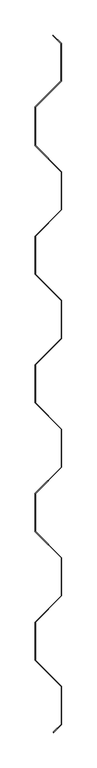
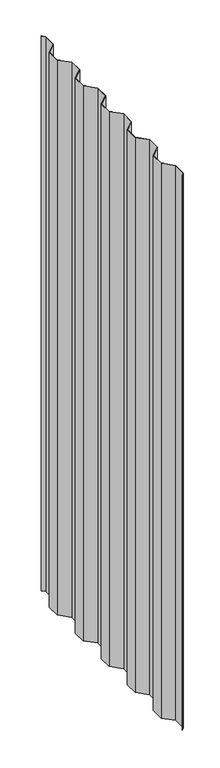
"""IFC4 building model written with IfcOpenShell, lengths in millimetres: proxy geometry, MBCI 7.2-V Panel7 : MBCI 7.2-V Panel-1."""

from ifc_helpers import new_model, si_unit, frame, origin, place, context, project, spatial, polyline, outline, extrude, source, transform, mapped, element, save


def generic_models_abe479ed(model_context):
    return source(origin(), model_context, "Body", "SweptSolid", [
        extrude(outline(polyline([(587365.8648989, -532709.4731976), (587365.8648989, -532763.5849068), (587354.4642648, -532774.9855409), (587354.4223399, -532774.1855668), (587365.2695864, -532763.3383203), (587365.2695864, -532709.7197841), (587327.7791864, -532672.2293841), (587327.7791864, -532617.9487203), (587365.2695864, -532580.4583203), (587365.2695864, -532526.8397841), (587327.7791864, -532489.3493841), (587327.7791864, -532435.0687203), (587365.2695864, -532397.5783203), (587365.2695864, -532343.9597841), (587327.7791864, -532306.4693841), (587327.7791864, -532252.1887203), (587365.2695864, -532214.6983203), (587365.2695864, -532161.0797841), (587327.7791864, -532123.5893841), (587327.7791864, -532069.3087203), (587365.2695864, -532031.8183203), (587365.2695864, -531978.1997841), (587327.7791864, -531940.7093841), (587327.7791864, -531885.5651203), (587364.6599864, -531848.6843203), (587364.6599864, -531795.5961933), (587353.5295525, -531784.4657594), (587353.5845762, -531783.6788841), (587365.2552989, -531795.3496068), (587365.2552989, -531848.9309068), (587328.3744989, -531885.8117068), (587328.3744989, -531940.4627976), (587365.8648989, -531977.9531976), (587365.8648989, -532032.0649068), (587328.3744989, -532069.5553068), (587328.3744989, -532123.3427976), (587365.8648989, -532160.8331976), (587365.8648989, -532214.9449068), (587328.3744989, -532252.4353068), (587328.3744989, -532306.2227976), (587365.8648989, -532343.7131976), (587365.8648989, -532397.8249068), (587328.3744989, -532435.3153068), (587328.3744989, -532489.1027976), (587365.8648989, -532526.5931976), (587365.8648989, -532580.7049068), (587328.3744989, -532618.1953068), (587328.3744989, -532671.9827976), (587365.8648989, -532709.4731976)])), frame((0.0, 0.0, 51.59375), z_axis=(0.0, 0.0, 1.0), x_axis=(1.0, 0.0, 0.0)), (0.0, 0.0, 1.0), 2386.80625),
    ])


if __name__ == "__main__":
    model = new_model("IFC4")
    model_context = context("Model", 3, world=origin())
    ifc_project = project(units=[si_unit("LENGTHUNIT", "METRE", prefix="MILLI")], contexts=[model_context])
    site = spatial("IfcSite", under=ifc_project)
    building = spatial("IfcBuilding", under=site)
    placement = place(None, origin())
    generic_models_shape = generic_models_abe479ed(model_context)
    element("IfcBuildingElementProxy", 1, Name="MBCI 7.2-V Panel7 : MBCI 7.2-V Panel-1", ObjectType="MBCI 7.2-V Panel7 : MBCI 7.2-V Panel-1", at=placement, inside=building, context=model_context, shape_type="MappedRepresentation", body=[
        mapped(generic_models_shape, transform((0.0, 0.0, 0.0), x_axis=(1.0, 0.0, 0.0), y_axis=(0.0, 1.0, 0.0), z_axis=(0.0, 0.0, 1.0))),
    ])
    save(model, "model.ifc")

# Revit data of these elements
# Element 1 (IfcBuildingElementProxy, "MBCI 7.2-V Panel7 : MBCI 7.2-V Panel-1")
#   Materials on its faces: "MTL PANEL"
# Materials
#   "MTL PANEL": class "Generic", colour RGB 239 242 240, transparency 0, Cost = 0
